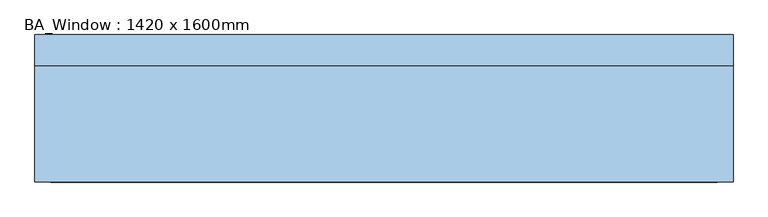
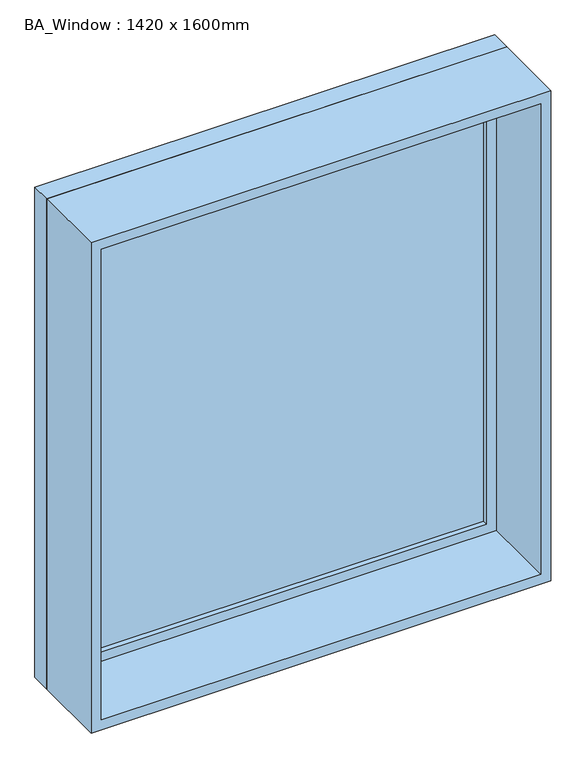
"""IFC4 building model written with IfcOpenShell, lengths in millimetres: window geometry, BA_Window : 1420 x 1600mm."""

from ifc_helpers import new_model, si_unit, frame, origin, place, context, project, spatial, polyline, outline, extrude, source, transform, mapped, element, save


def ba_window_1420_x_1600mm_ad9b87f8(model_context):
    return source(origin(), model_context, "Body", "SweptSolid", [
        extrude(outline(polyline([(-647.0, 128.0), (647.0, 128.0), (647.0, 116.0), (-647.0, 116.0), (-647.0, 128.0)])), frame((0.0, 0.0, 978.0), z_axis=(0.0, 0.0, 1.0), x_axis=(1.0, 0.0, 0.0)), (0.0, 0.0, 1.0), 1474.0),
        extrude(outline(polyline([(2496.0, -691.0), (934.0, -691.0), (934.0, 691.0), (2496.0, 691.0), (2496.0, -691.0)]), holes=[polyline([(2452.0, -647.0), (2452.0, 647.0), (978.0, 647.0), (978.0, -647.0), (2452.0, -647.0)])]), frame((0.0, 100.0, 0.0), z_axis=(0.0, 1.0, 0.0), x_axis=(0.0, 0.0, 1.0)), (0.0, 0.0, 1.0), 44.0),
        extrude(outline(polyline([(2515.0, -710.0), (915.0, -710.0), (915.0, 710.0), (2515.0, 710.0), (2515.0, -710.0)]), holes=[polyline([(2496.0, -691.0), (2496.0, 691.0), (934.0, 691.0), (934.0, -691.0), (2496.0, -691.0)])]), frame((0.0, 100.0, 0.0), z_axis=(0.0, 1.0, 0.0), x_axis=(0.0, 0.0, 1.0)), (0.0, 0.0, 1.0), 63.0),
        extrude(outline(polyline([(2515.0, -710.0), (915.0, -710.0), (915.0, 710.0), (2515.0, 710.0), (2515.0, -710.0)]), holes=[polyline([(2483.0, -678.0), (2483.0, 678.0), (947.0, 678.0), (947.0, -678.0), (2483.0, -678.0)])]), frame((0.0, -137.0, 0.0), z_axis=(0.0, 1.0, 0.0), x_axis=(0.0, 0.0, 1.0)), (0.0, 0.0, 1.0), 237.0),
    ])


if __name__ == "__main__":
    model = new_model("IFC4")
    model_context = context("Model", 3, world=origin())
    ifc_project = project(units=[si_unit("LENGTHUNIT", "METRE", prefix="MILLI")], contexts=[model_context])
    site = spatial("IfcSite", under=ifc_project)
    building = spatial("IfcBuilding", under=site)
    placement = place(None, origin())
    ba_window_1420_x_1600mm_shape = ba_window_1420_x_1600mm_ad9b87f8(model_context)
    element("IfcWindow", 1, ObjectType="BA_Window : 1420 x 1600mm", at=placement, inside=building, context=model_context, shape_type="MappedRepresentation", body=[
        mapped(ba_window_1420_x_1600mm_shape, transform((0.0, 0.0, 0.0), x_axis=(1.0, 0.0, 0.0), y_axis=(0.0, 1.0, 0.0), z_axis=(0.0, 0.0, 1.0))),
    ])
    save(model, "model.ifc")

# Revit data of these elements
# Type "BA_Window : 1420 x 1600mm"
#   Type Mark = "39"
#   Construction Type Id = "GSP4R"
#   Analytic Construction = "1/8 in Pilkington single glazing"
#   Visual Light Transmittance = 0.9
#   Thermal Resistance (R) = 0.271106 (m²·K)/W
#   Solar Heat Gain Coefficient = 0.78
#   Heat Transfer Coefficient (U) = 3.6886 W/(m²·K)
#   Height = 1600 mm
#   Default Sill Height = 915 mm
#   Width = 1420 mm
#   Window Inset = 19 mm
#   Define Thermal Properties by = 1
#   Frame Exterior Material = Default
#   Frame Interior Material = Default
#   Glass Pane Material = Glass
#   Sash = Default
#   Wall Closure = (empty or 0)
# Element 1 (IfcWindow, "BA_Window : 1420 x 1600mm")
#   Materials on its faces: "Default", "Glass"
# Materials
#   "Default": class "Generic", colour RGB 255 255 255, transparency 0, Cost = 0
#   "Glass": class "Glass", colour RGB 0 128 192, transparency 0.9, Description = "Soda Lime Glass", Cost = 0
